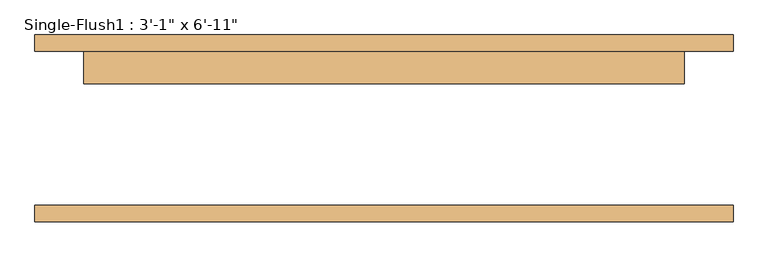
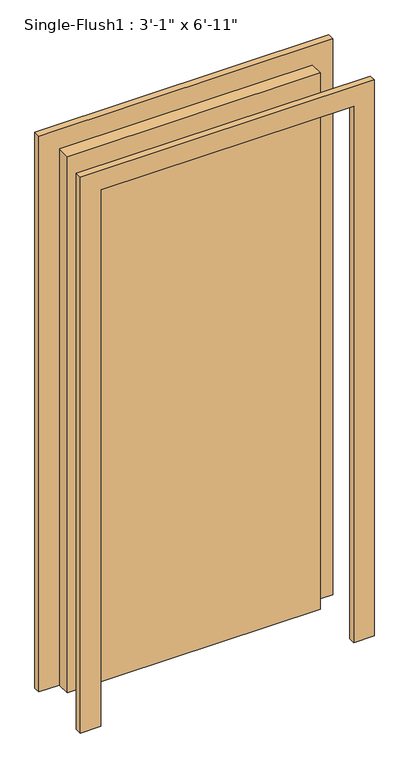
"""IFC4 building model written with IfcOpenShell, lengths in millimetres: door geometry."""

from ifc_helpers import new_model, si_unit, frame, origin, origin_with_axes, place, context, project, spatial, polyline, outline, extrude, source, transform, mapped, element, save


def door_4a887283(model_context):
    return source(origin(), model_context, "Body", "SweptSolid", [
        extrude(outline(polyline([(2184.4, -546.1), (0.0, -546.1), (0.0, -469.9), (2108.2, -469.9), (2108.2, 469.9), (0.0, 469.9), (0.0, 546.1), (2184.4, 546.1), (2184.4, -546.1)])), frame((0.0, 120.65, 0.0), z_axis=(0.0, 1.0, 0.0), x_axis=(0.0, 0.0, 1.0)), (0.0, 0.0, 1.0), 25.4),
        extrude(outline(polyline([(2184.4, 546.1), (2184.4, -546.1), (0.0, -546.1), (0.0, -469.9), (2108.2, -469.9), (2108.2, 469.9), (0.0, 469.9), (0.0, 546.1), (2184.4, 546.1)])), frame((0.0, -146.05, 0.0), z_axis=(0.0, 1.0, 0.0), x_axis=(0.0, 0.0, 1.0)), (0.0, 0.0, 1.0), 25.4),
        extrude(outline(polyline([(469.9, 69.85), (-469.9, 69.85), (-469.9, 120.65), (469.9, 120.65), (469.9, 69.85)])), origin_with_axes(), (0.0, 0.0, 1.0), 2108.2),
    ])


if __name__ == "__main__":
    model = new_model("IFC4")
    model_context = context("Model", 3, world=origin())
    ifc_project = project(units=[si_unit("LENGTHUNIT", "METRE", prefix="MILLI")], contexts=[model_context])
    site = spatial("IfcSite", under=ifc_project)
    building = spatial("IfcBuilding", under=site)
    placement = place(None, origin())
    door_shape = door_4a887283(model_context)
    element("IfcDoor", 1, ObjectType="Single-Flush1 : 3'-1\" x 6'-11\"", at=placement, inside=building, context=model_context, shape_type="MappedRepresentation", body=[
        mapped(door_shape, transform((0.0, 0.0, 0.0), x_axis=(1.0, 0.0, 0.0), y_axis=(0.0, 1.0, 0.0), z_axis=(0.0, 0.0, 1.0))),
    ])
    save(model, "model.ifc")

# Revit data of these elements
# Type "Single-Flush1 : 3'-1\" x 6'-11\""
#   Type Mark = "27"
#   Construction Type Id = "MDOOR"
#   Assembly Code = "C1020"
#   Analytic Construction = "Metal"
#   Thickness = 0' - 2"
#   Heat Transfer Coefficient (U) = 3.7021 W/(m²·K)
#   Height = 6' - 11"
#   Trim Projection Ext = 0' - 1"
#   Trim Projection Int = 0' - 1"
#   Trim Width = 0' - 3"
#   Width = 3' - 1"
#   Door Material = Door - Panel
#   Frame Material = Door - Frame
#   Visual Light Transmittance = 0
#   Solar Heat Gain Coefficient = 0
#   Function = (empty or 0)
#   Wall Closure = (empty or 0)
# Element 1 (IfcDoor, "Single-Flush1 : 3'-1\" x 6'-11\"")
#   Materials on its faces: "Door - Frame", "Door - Panel"
# Materials
#   "Door - Panel": class "Wood", colour RGB 210 159 95, transparency 0, Cost = 0
#   "Door - Frame": class "Miscellaneous", colour RGB 118 70 51, transparency 0, Cost = 0
